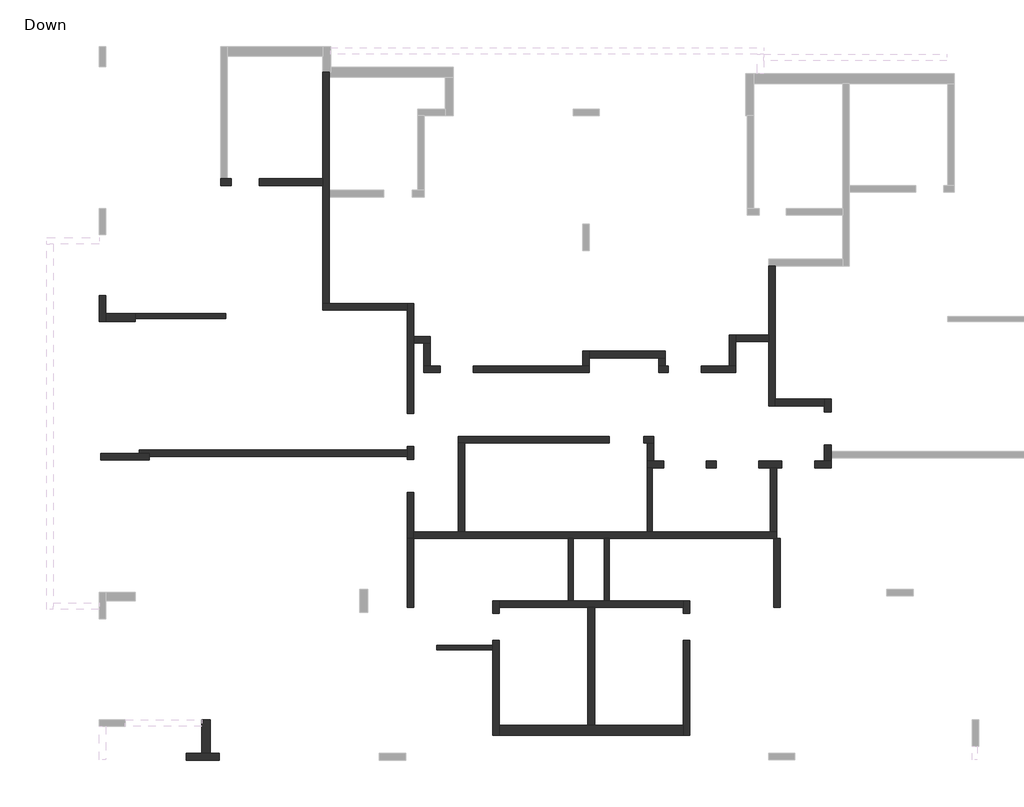
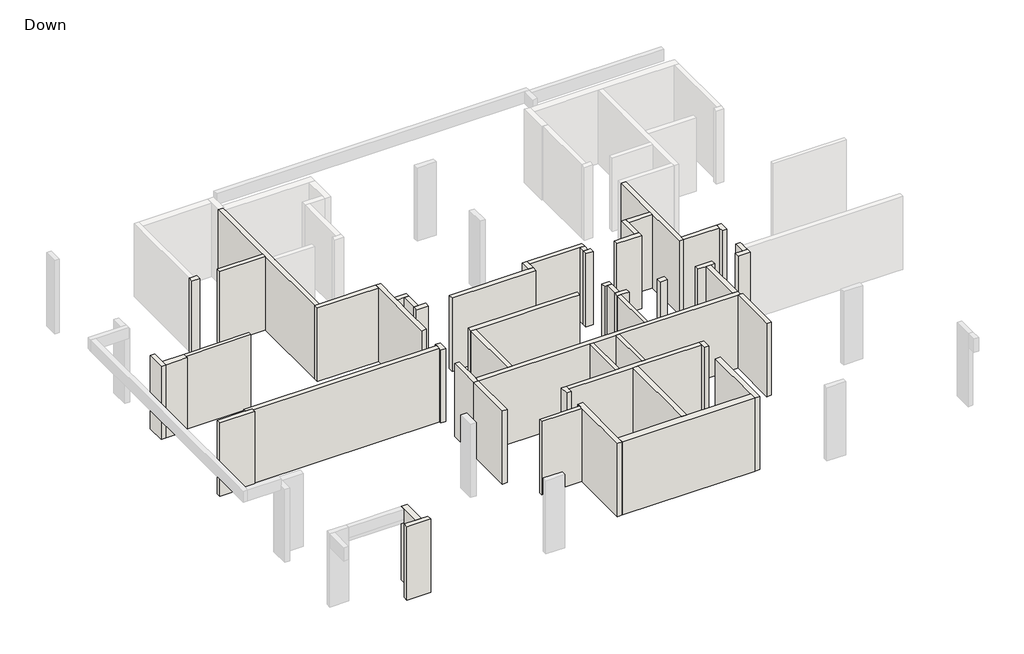
# One storey, part 1 of 2: 52 walls.
# Revit data of these elements (continued)
# Element 4 (IfcWall, "15")
#   Comments = ""
#   Mark = "W73"
#   SOFiSTiK_EdgeZones = "W75"
#   SOFiSTiK_AMG_Comments = ""
#   Top Offset = 0 cm
#   Base Offset = 0 cm
#   wall height = 327 cm
#   SOFiSTiK_AMG_Scheduled = yes
#   SOFiSTiK_AMG_Adjusted = yes
#   Phase Created = New Construction
#   Base Constraint = Down
#   Top Constraint = Typical Floor
#   Materials on its faces: "Concrete"
# Element 5 (IfcWall, "15")
#   Comments = ""
#   Mark = "W75"
#   SOFiSTiK_EdgeZones = "W77"
#   SOFiSTiK_AMG_Comments = ""
#   Top Offset = 0 cm
#   Base Offset = 0 cm
#   wall height = 327 cm
#   SOFiSTiK_AMG_Scheduled = yes
#   SOFiSTiK_AMG_Adjusted = yes
#   Phase Created = New Construction
#   Base Constraint = Down
#   Top Constraint = Typical Floor
#   Materials on its faces: "Concrete"
# Element 6 (IfcWall, "20")
#   Comments = ""
#   Mark = "W1"
#   SOFiSTiK_EdgeZones = "W1"
#   SOFiSTiK_AMG_Comments = ""
#   Top Offset = 0 cm
#   Base Offset = 0 cm
#   wall height = 327 cm
#   SOFiSTiK_AMG_Scheduled = yes
#   SOFiSTiK_AMG_Adjusted = yes
#   Phase Created = New Construction
#   Base Constraint = Down
#   Top Constraint = Typical Floor
#   Materials on its faces: "Concrete"
# Element 7 (IfcWall, "20")
#   Comments = ""
#   Mark = "W2"
#   SOFiSTiK_EdgeZones = "W2"
#   SOFiSTiK_AMG_Comments = ""
#   Top Offset = 0 cm
#   Base Offset = 0 cm
#   wall height = 327 cm
#   SOFiSTiK_AMG_Scheduled = yes
#   SOFiSTiK_AMG_Adjusted = yes
#   Phase Created = New Construction
#   Base Constraint = Down
#   Top Constraint = Typical Floor
#   Materials on its faces: "Concrete"
# Element 8 (IfcWall, "20")
#   Comments = ""
#   Mark = "W3"
#   SOFiSTiK_EdgeZones = "W3"
#   SOFiSTiK_AMG_Comments = ""
#   Top Offset = 0 cm
#   Base Offset = 0 cm
#   wall height = 327 cm
#   SOFiSTiK_AMG_Scheduled = yes
#   SOFiSTiK_AMG_Adjusted = yes
#   Phase Created = New Construction
#   Base Constraint = Down
#   Top Constraint = Typical Floor
#   Materials on its faces: "Concrete"
# Element 9 (IfcWall, "20")
#   Comments = ""
#   Mark = "W4"
#   SOFiSTiK_EdgeZones = "W5"
#   SOFiSTiK_AMG_Comments = ""
#   Top Offset = 0 cm
#   Base Offset = 0 cm
#   wall height = 327 cm
#   SOFiSTiK_AMG_Scheduled = yes
#   SOFiSTiK_AMG_Adjusted = yes
#   Phase Created = New Construction
#   Base Constraint = Down
#   Top Constraint = Typical Floor
#   Materials on its faces: "Concrete"
# Element 10 (IfcWall, "20")
#   Comments = ""
#   Mark = "W5"
#   SOFiSTiK_EdgeZones = "W6"
#   SOFiSTiK_AMG_Comments = ""
#   Top Offset = 0 cm
#   Base Offset = 0 cm
#   wall height = 327 cm
#   SOFiSTiK_AMG_Scheduled = yes
#   SOFiSTiK_AMG_Adjusted = yes
#   Phase Created = New Construction
#   Base Constraint = Down
#   Top Constraint = Typical Floor
#   Materials on its faces: "Concrete"
# Element 11 (IfcWall, "20")
#   Comments = ""
#   Mark = "W6"
#   SOFiSTiK_EdgeZones = "W7"
#   SOFiSTiK_AMG_Comments = ""
#   Top Offset = 0 cm
#   Base Offset = 0 cm
#   wall height = 327 cm
#   SOFiSTiK_AMG_Scheduled = yes
#   SOFiSTiK_AMG_Adjusted = yes
#   Phase Created = New Construction
#   Base Constraint = Down
#   Top Constraint = Typical Floor
#   Materials on its faces: "Concrete"
# Element 12 (IfcWall, "20")
#   Comments = ""
#   Mark = "W7"
#   SOFiSTiK_EdgeZones = "W8"
#   SOFiSTiK_AMG_Comments = ""
#   Top Offset = 0 cm
#   Base Offset = 0 cm
#   wall height = 327 cm
#   SOFiSTiK_AMG_Scheduled = yes
#   SOFiSTiK_AMG_Adjusted = yes
#   Phase Created = New Construction
#   Base Constraint = Down
#   Top Constraint = Typical Floor
#   Materials on its faces: "Concrete"
# Element 13 (IfcWall, "20")
#   Comments = ""
#   Mark = "W9"
#   SOFiSTiK_EdgeZones = "W10"
#   SOFiSTiK_AMG_Comments = ""
#   Top Offset = 0 cm
#   Base Offset = 0 cm
#   wall height = 327 cm
#   SOFiSTiK_AMG_Scheduled = yes
#   SOFiSTiK_AMG_Adjusted = yes
#   Phase Created = New Construction
#   Base Constraint = Down
#   Top Constraint = Typical Floor
#   Materials on its faces: "Concrete"
# Element 14 (IfcWall, "20")
#   Comments = ""
#   Mark = "W14"
#   SOFiSTiK_EdgeZones = "W15"
#   SOFiSTiK_AMG_Comments = ""
#   Top Offset = 0 cm
#   Base Offset = 0 cm
#   wall height = 327 cm
#   SOFiSTiK_AMG_Scheduled = yes
#   SOFiSTiK_AMG_Adjusted = yes
#   Phase Created = New Construction
#   Base Constraint = Down
#   Top Constraint = Typical Floor
#   Materials on its faces: "Concrete"
# Element 15 (IfcWall, "20")
#   Comments = ""
#   Mark = "W15"
#   SOFiSTiK_EdgeZones = "W16"
#   SOFiSTiK_AMG_Comments = ""
#   Top Offset = 0 cm
#   Base Offset = 0 cm
#   wall height = 327 cm
#   SOFiSTiK_AMG_Scheduled = yes
#   SOFiSTiK_AMG_Adjusted = yes
#   Phase Created = New Construction
#   Base Constraint = Down
#   Top Constraint = Typical Floor
#   Materials on its faces: "Concrete"
# Element 16 (IfcWall, "20")
#   Comments = ""
#   Mark = "W16"
#   SOFiSTiK_EdgeZones = "W17"
#   SOFiSTiK_AMG_Comments = ""
#   Top Offset = 0 cm
#   Base Offset = 0 cm
#   wall height = 327 cm
#   SOFiSTiK_AMG_Scheduled = yes
#   SOFiSTiK_AMG_Adjusted = yes
#   Phase Created = New Construction
#   Base Constraint = Down
#   Top Constraint = Typical Floor
#   Materials on its faces: "Concrete"
# Element 17 (IfcWall, "20")
#   Comments = ""
#   Mark = "W17"
#   SOFiSTiK_EdgeZones = "W18"
#   SOFiSTiK_AMG_Comments = ""
#   Top Offset = 0 cm
#   Base Offset = 0 cm
#   wall height = 327 cm
#   SOFiSTiK_AMG_Scheduled = yes
#   SOFiSTiK_AMG_Adjusted = yes
#   Phase Created = New Construction
#   Base Constraint = Down
#   Top Constraint = Typical Floor
#   Materials on its faces: "Concrete"
# Element 18 (IfcWall, "20")
#   Comments = ""
#   Mark = "W18"
#   SOFiSTiK_EdgeZones = "W19"
#   SOFiSTiK_AMG_Comments = ""
#   Top Offset = 0 cm
#   Base Offset = 0 cm
#   wall height = 327 cm
#   SOFiSTiK_AMG_Scheduled = yes
#   SOFiSTiK_AMG_Adjusted = yes
#   Phase Created = New Construction
#   Base Constraint = Down
#   Top Constraint = Typical Floor
#   Materials on its faces: "Concrete"
# Element 19 (IfcWall, "20")
#   Comments = ""
#   Mark = "W19"
#   SOFiSTiK_EdgeZones = "W20"
#   SOFiSTiK_AMG_Comments = ""
#   Top Offset = 0 cm
#   Base Offset = 0 cm
#   wall height = 327 cm
#   SOFiSTiK_AMG_Scheduled = yes
#   SOFiSTiK_AMG_Adjusted = yes
#   Phase Created = New Construction
#   Base Constraint = Down
#   Top Constraint = Typical Floor
#   Materials on its faces: "Concrete"
# Element 20 (IfcWall, "20")
#   Comments = ""
#   Mark = "W20"
#   SOFiSTiK_EdgeZones = "W21"
#   SOFiSTiK_AMG_Comments = ""
#   Top Offset = 0 cm
#   Base Offset = 0 cm
#   wall height = 327 cm
#   SOFiSTiK_AMG_Scheduled = yes
#   SOFiSTiK_AMG_Adjusted = yes
#   Phase Created = New Construction
#   Base Constraint = Down
#   Top Constraint = Typical Floor
#   Materials on its faces: "Concrete"
# Element 21 (IfcWall, "20")
#   Comments = ""
#   Mark = "W21"
#   SOFiSTiK_EdgeZones = "W22"
#   SOFiSTiK_AMG_Comments = ""
#   Top Offset = 0 cm
#   Base Offset = 0 cm
#   wall height = 327 cm
#   SOFiSTiK_AMG_Scheduled = yes
#   SOFiSTiK_AMG_Adjusted = yes
#   Phase Created = New Construction
#   Base Constraint = Down
#   Top Constraint = Typical Floor
#   Materials on its faces: "Concrete"
# Element 22 (IfcWall, "20")
#   Comments = ""
#   Mark = "W22"
#   SOFiSTiK_EdgeZones = "W23"
#   SOFiSTiK_AMG_Comments = ""
#   Top Offset = 0 cm
#   Base Offset = 0 cm
#   wall height = 327 cm
#   SOFiSTiK_AMG_Scheduled = yes
#   SOFiSTiK_AMG_Adjusted = yes
#   Phase Created = New Construction
#   Base Constraint = Down
#   Top Constraint = Typical Floor
#   Materials on its faces: "Concrete"
# Element 23 (IfcWall, "20")
#   Comments = ""
#   Mark = "W23"
#   SOFiSTiK_EdgeZones = "W24"
#   SOFiSTiK_AMG_Comments = ""
#   Top Offset = 0 cm
#   Base Offset = 0 cm
#   wall height = 327 cm
#   SOFiSTiK_AMG_Scheduled = yes
#   SOFiSTiK_AMG_Adjusted = yes
#   Phase Created = New Construction
#   Base Constraint = Down
#   Top Constraint = Typical Floor
#   Materials on its faces: "Concrete"
# Element 24 (IfcWall, "20")
#   Comments = ""
#   Mark = "W24"
#   SOFiSTiK_EdgeZones = "W25"
#   SOFiSTiK_AMG_Comments = ""
#   Top Offset = 0 cm
#   Base Offset = 0 cm
#   wall height = 327 cm
#   SOFiSTiK_AMG_Scheduled = yes
#   SOFiSTiK_AMG_Adjusted = yes
#   Phase Created = New Construction
#   Base Constraint = Down
#   Top Constraint = Typical Floor
#   Materials on its faces: "Concrete"
# Element 25 (IfcWall, "20")
#   Comments = ""
#   Mark = "W25"
#   SOFiSTiK_EdgeZones = "W26"
#   SOFiSTiK_AMG_Comments = ""
#   Top Offset = 0 cm
#   Base Offset = 0 cm
#   wall height = 327 cm
#   SOFiSTiK_AMG_Scheduled = yes
#   SOFiSTiK_AMG_Adjusted = yes
#   Phase Created = New Construction
#   Base Constraint = Down
#   Top Constraint = Typical Floor
#   Materials on its faces: "Concrete"
# Element 26 (IfcWall, "20")
#   Comments = ""
#   Mark = "W26"
#   SOFiSTiK_EdgeZones = "W27"
#   SOFiSTiK_AMG_Comments = ""
#   Top Offset = 0 cm
#   Base Offset = 0 cm
#   wall height = 327 cm
#   SOFiSTiK_AMG_Scheduled = yes
#   SOFiSTiK_AMG_Adjusted = yes
#   Phase Created = New Construction
#   Base Constraint = Down
#   Top Constraint = Typical Floor
#   Materials on its faces: "Concrete"
# Element 27 (IfcWall, "20")
#   Comments = ""
#   Mark = "W27"
#   SOFiSTiK_EdgeZones = "W28"
#   SOFiSTiK_AMG_Comments = ""
#   Top Offset = 0 cm
#   Base Offset = 0 cm
#   wall height = 327 cm
#   SOFiSTiK_AMG_Scheduled = yes
#   SOFiSTiK_AMG_Adjusted = yes
#   Phase Created = New Construction
#   Base Constraint = Down
#   Top Constraint = Typical Floor
#   Materials on its faces: "Concrete"
# Element 28 (IfcWall, "20")
#   Comments = ""
#   Mark = "W28"
#   SOFiSTiK_EdgeZones = "W29"
#   SOFiSTiK_AMG_Comments = ""
#   Top Offset = 0 cm
#   Base Offset = 0 cm
#   wall height = 327 cm
#   SOFiSTiK_AMG_Scheduled = yes
#   SOFiSTiK_AMG_Adjusted = yes
#   Phase Created = New Construction
#   Base Constraint = Down
#   Top Constraint = Typical Floor
#   Materials on its faces: "Concrete"
# Element 29 (IfcWall, "20")
#   Comments = ""
#   Mark = "W29"
#   SOFiSTiK_EdgeZones = "W30"
#   SOFiSTiK_AMG_Comments = ""
#   Top Offset = 0 cm
#   Base Offset = 0 cm
#   wall height = 327 cm
#   SOFiSTiK_AMG_Scheduled = yes
#   SOFiSTiK_AMG_Adjusted = yes
#   Phase Created = New Construction
#   Base Constraint = Down
#   Top Constraint = Typical Floor
#   Materials on its faces: "Concrete"
# Element 30 (IfcWall, "20")
#   Comments = ""
#   Mark = "W30"
#   SOFiSTiK_EdgeZones = "W32"
#   SOFiSTiK_AMG_Comments = ""
#   Top Offset = 0 cm
#   Base Offset = 0 cm
#   wall height = 327 cm
#   SOFiSTiK_AMG_Scheduled = yes
#   SOFiSTiK_AMG_Adjusted = yes
#   Phase Created = New Construction
#   Base Constraint = Down
#   Top Constraint = Typical Floor
#   Materials on its faces: "Concrete"
# Element 31 (IfcWall, "20")
#   Comments = ""
#   Mark = "W31"
#   SOFiSTiK_EdgeZones = "W33"
#   SOFiSTiK_AMG_Comments = ""
#   Top Offset = 0 cm
#   Base Offset = 0 cm
#   wall height = 327 cm
#   SOFiSTiK_AMG_Scheduled = yes
#   SOFiSTiK_AMG_Adjusted = yes
#   Phase Created = New Construction
#   Base Constraint = Down
#   Top Constraint = Typical Floor
#   Materials on its faces: "Concrete"
# Element 32 (IfcWall, "20")
#   Comments = ""
#   Mark = "W32"
#   SOFiSTiK_EdgeZones = "W34"
#   SOFiSTiK_AMG_Comments = ""
#   Top Offset = 0 cm
#   Base Offset = 0 cm
#   wall height = 327 cm
#   SOFiSTiK_AMG_Scheduled = yes
#   SOFiSTiK_AMG_Adjusted = yes
#   Phase Created = New Construction
#   Base Constraint = Down
#   Top Constraint = Typical Floor
#   Materials on its faces: "Concrete"
# Element 33 (IfcWall, "20")
#   Comments = ""
#   Mark = "W33"
#   SOFiSTiK_EdgeZones = "W35"
#   SOFiSTiK_AMG_Comments = ""
#   Top Offset = 0 cm
#   Base Offset = 0 cm
#   wall height = 327 cm
#   SOFiSTiK_AMG_Scheduled = yes
#   SOFiSTiK_AMG_Adjusted = yes
#   Phase Created = New Construction
#   Base Constraint = Down
#   Top Constraint = Typical Floor
#   Materials on its faces: "Concrete"
# Element 34 (IfcWall, "20")
#   Comments = ""
#   Mark = "W34"
#   SOFiSTiK_EdgeZones = "W36"
#   SOFiSTiK_AMG_Comments = ""
#   Top Offset = 0 cm
#   Base Offset = 0 cm
#   wall height = 327 cm
#   SOFiSTiK_AMG_Scheduled = yes
#   SOFiSTiK_AMG_Adjusted = yes
#   Phase Created = New Construction
#   Base Constraint = Down
#   Top Constraint = Typical Floor
#   Materials on its faces: "Concrete"
# Element 35 (IfcWall, "20")
#   Comments = ""
#   Mark = "W35"
#   SOFiSTiK_EdgeZones = "W37"
#   SOFiSTiK_AMG_Comments = ""
#   Top Offset = 0 cm
#   Base Offset = 0 cm
#   wall height = 327 cm
#   SOFiSTiK_AMG_Scheduled = yes
#   SOFiSTiK_AMG_Adjusted = yes
#   Phase Created = New Construction
#   Base Constraint = Down
#   Top Constraint = Typical Floor
#   Materials on its faces: "Concrete"
# Element 36 (IfcWall, "20")
#   Comments = ""
#   Mark = "W36"
#   SOFiSTiK_EdgeZones = "W38"
#   SOFiSTiK_AMG_Comments = ""
#   Top Offset = 0 cm
#   Base Offset = 0 cm
#   wall height = 327 cm
#   SOFiSTiK_AMG_Scheduled = yes
#   SOFiSTiK_AMG_Adjusted = yes
#   Phase Created = New Construction
#   Base Constraint = Down
#   Top Constraint = Typical Floor
#   Materials on its faces: "Concrete"
# Element 37 (IfcWall, "20")
#   Comments = ""
#   Mark = "W37"
#   SOFiSTiK_EdgeZones = "W39"
#   SOFiSTiK_AMG_Comments = ""
#   Top Offset = 0 cm
#   Base Offset = 0 cm
#   wall height = 327 cm
#   SOFiSTiK_AMG_Scheduled = yes
#   SOFiSTiK_AMG_Adjusted = yes
#   Phase Created = New Construction
#   Base Constraint = Down
#   Top Constraint = Typical Floor
#   Materials on its faces: "Concrete"
# Element 38 (IfcWall, "20")
#   Comments = ""
#   Mark = "W38"
#   SOFiSTiK_EdgeZones = "W40"
#   SOFiSTiK_AMG_Comments = ""
#   Top Offset = 0 cm
#   Base Offset = 0 cm
#   wall height = 327 cm
#   SOFiSTiK_AMG_Scheduled = yes
#   SOFiSTiK_AMG_Adjusted = yes
#   Phase Created = New Construction
#   Base Constraint = Down
#   Top Constraint = Typical Floor
#   Materials on its faces: "Concrete"
# Element 39 (IfcWall, "20")
#   Comments = ""
#   Mark = "W39"
#   SOFiSTiK_EdgeZones = "W41"
#   SOFiSTiK_AMG_Comments = ""
#   Top Offset = 0 cm
#   Base Offset = 0 cm
#   wall height = 327 cm
#   SOFiSTiK_AMG_Scheduled = yes
#   SOFiSTiK_AMG_Adjusted = yes
#   Phase Created = New Construction
#   Base Constraint = Down
#   Top Constraint = Typical Floor
#   Materials on its faces: "Concrete"
# Element 40 (IfcWall, "20")
#   Comments = ""
#   Mark = "W40"
#   SOFiSTiK_EdgeZones = "W42"
#   SOFiSTiK_AMG_Comments = ""
#   Top Offset = 0 cm
#   Base Offset = 0 cm
#   wall height = 327 cm
#   SOFiSTiK_AMG_Scheduled = yes
#   SOFiSTiK_AMG_Adjusted = yes
#   Phase Created = New Construction
#   Base Constraint = Down
#   Top Constraint = Typical Floor
#   Materials on its faces: "Concrete"
# Element 41 (IfcWall, "20")
#   Comments = ""
#   Mark = "W41"
#   SOFiSTiK_EdgeZones = "W43"
#   SOFiSTiK_AMG_Comments = ""
#   Top Offset = 0 cm
#   Base Offset = 0 cm
#   wall height = 327 cm
#   SOFiSTiK_AMG_Scheduled = yes
#   SOFiSTiK_AMG_Adjusted = yes
#   Phase Created = New Construction
#   Base Constraint = Down
#   Top Constraint = Typical Floor
#   Materials on its faces: "Concrete"
# Element 42 (IfcWall, "20")
#   Comments = ""
#   Mark = "W42"
#   SOFiSTiK_EdgeZones = "W44"
#   SOFiSTiK_AMG_Comments = ""
#   Top Offset = 0 cm
#   Base Offset = 0 cm
#   wall height = 327 cm
#   SOFiSTiK_AMG_Scheduled = yes
#   SOFiSTiK_AMG_Adjusted = yes
#   Phase Created = New Construction
#   Base Constraint = Down
#   Top Constraint = Typical Floor
#   Materials on its faces: "Concrete"
# Element 43 (IfcWall, "20")
#   Comments = ""
#   Mark = "W51"
#   SOFiSTiK_EdgeZones = "W53"
#   SOFiSTiK_AMG_Comments = ""
#   Top Offset = 0 cm
#   Base Offset = 0 cm
#   wall height = 327 cm
#   SOFiSTiK_AMG_Scheduled = yes
#   SOFiSTiK_AMG_Adjusted = yes
#   Phase Created = New Construction
#   Base Constraint = Down
#   Top Constraint = Typical Floor
#   Materials on its faces: "Concrete"
# Element 44 (IfcWall, "20")
#   Comments = ""
#   Mark = "W52"
#   SOFiSTiK_EdgeZones = "W54"
#   SOFiSTiK_AMG_Comments = ""
#   Top Offset = 0 cm
#   Base Offset = 0 cm
#   wall height = 327 cm
#   SOFiSTiK_AMG_Scheduled = yes
#   SOFiSTiK_AMG_Adjusted = yes
#   Phase Created = New Construction
#   Base Constraint = Down
#   Top Constraint = Typical Floor
#   Materials on its faces: "Concrete"
# Element 45 (IfcWall, "20")
#   Comments = ""
#   Mark = "W53"
#   SOFiSTiK_EdgeZones = "W55"
#   SOFiSTiK_AMG_Comments = ""
#   Top Offset = 0 cm
#   Base Offset = 0 cm
#   wall height = 327 cm
#   SOFiSTiK_AMG_Scheduled = yes
#   SOFiSTiK_AMG_Adjusted = yes
#   Phase Created = New Construction
#   Base Constraint = Down
#   Top Constraint = Typical Floor
#   Materials on its faces: "Concrete"
# Element 46 (IfcWall, "20")
#   Comments = ""
#   Mark = "W54"
#   SOFiSTiK_EdgeZones = "W56"
#   SOFiSTiK_AMG_Comments = ""
#   Top Offset = 0 cm
#   Base Offset = 0 cm
#   wall height = 327 cm
#   SOFiSTiK_AMG_Scheduled = yes
#   SOFiSTiK_AMG_Adjusted = yes
#   Phase Created = New Construction
#   Base Constraint = Down
#   Top Constraint = Typical Floor
#   Materials on its faces: "Concrete"
# Element 47 (IfcWall, "20")
#   Comments = ""
#   Mark = "W55"
#   SOFiSTiK_EdgeZones = "W57"
#   SOFiSTiK_AMG_Comments = ""
#   Top Offset = 0 cm
#   Base Offset = 0 cm
#   wall height = 327 cm
#   SOFiSTiK_AMG_Scheduled = yes
#   SOFiSTiK_AMG_Adjusted = yes
#   Phase Created = New Construction
#   Base Constraint = Down
#   Top Constraint = Typical Floor
#   Materials on its faces: "Concrete"
# Element 48 (IfcWall, "20")
#   Comments = ""
#   Mark = "W59"
#   SOFiSTiK_EdgeZones = "W61"
#   SOFiSTiK_AMG_Comments = ""
#   Top Offset = 0 cm
#   Base Offset = 0 cm
#   wall height = 327 cm
#   SOFiSTiK_AMG_Scheduled = yes
#   SOFiSTiK_AMG_Adjusted = yes
#   Phase Created = New Construction
#   Base Constraint = Down
#   Top Constraint = Typical Floor
#   Materials on its faces: "Concrete"
# Element 49 (IfcWall, "20")
#   Comments = ""
#   Mark = "W60"
#   SOFiSTiK_EdgeZones = "W62"
#   SOFiSTiK_AMG_Comments = ""
#   Top Offset = 0 cm
#   Base Offset = 0 cm
#   wall height = 327 cm
#   SOFiSTiK_AMG_Scheduled = yes
#   SOFiSTiK_AMG_Adjusted = yes
#   Phase Created = New Construction
#   Base Constraint = Down
#   Top Constraint = Typical Floor
#   Materials on its faces: "Concrete"
# Element 50 (IfcWall, "25")
#   Comments = ""
#   Mark = "W68"
#   SOFiSTiK_EdgeZones = "W70"
#   SOFiSTiK_AMG_Comments = ""
#   Top Offset = 0 cm
#   Base Offset = 0 cm
#   wall height = 327 cm
#   SOFiSTiK_AMG_Scheduled = yes
#   SOFiSTiK_AMG_Adjusted = yes
#   Phase Created = New Construction
#   Base Constraint = Down
#   Top Constraint = Typical Floor
#   Materials on its faces: "Concrete"
# Element 51 (IfcWall, "25")
#   Comments = ""
#   Mark = "W69"
#   SOFiSTiK_EdgeZones = "W71"
#   SOFiSTiK_AMG_Comments = ""
#   Top Offset = 0 cm
#   Base Offset = 0 cm
#   wall height = 327 cm
#   SOFiSTiK_AMG_Scheduled = yes
#   SOFiSTiK_AMG_Adjusted = yes
#   Phase Created = New Construction
#   Base Constraint = Down
#   Top Constraint = Typical Floor
#   Materials on its faces: "Concrete"
# Element 52 (IfcWall, "30")
#   Comments = ""
#   Mark = "W63"
#   SOFiSTiK_EdgeZones = "W65"
#   SOFiSTiK_AMG_Comments = ""
#   Top Offset = 0 cm
#   Base Offset = 0 cm
#   wall height = 327 cm
#   SOFiSTiK_AMG_Scheduled = yes
#   SOFiSTiK_AMG_Adjusted = yes
#   Phase Created = New Construction
#   Base Constraint = Down
#   Top Constraint = Typical Floor
#   Materials on its faces: "Concrete"
# Materials
#   "Concrete": class "Concrete", colour RGB 192 192 192, transparency 0, Keynote = "01000", Description = "Cast-in-place concrete", Cost = 0
